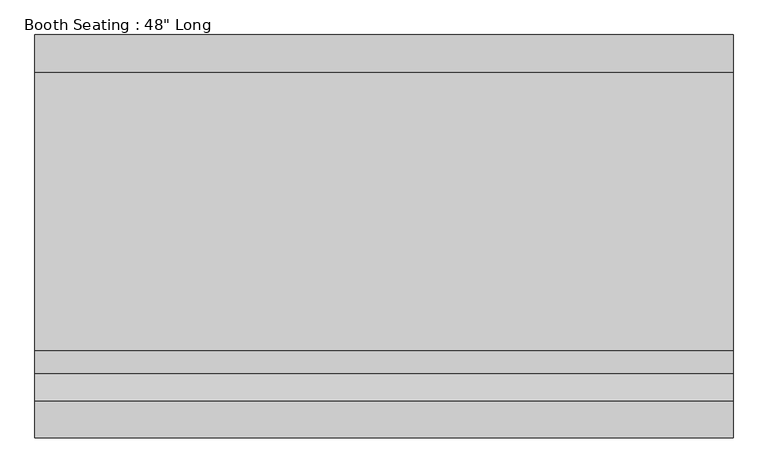
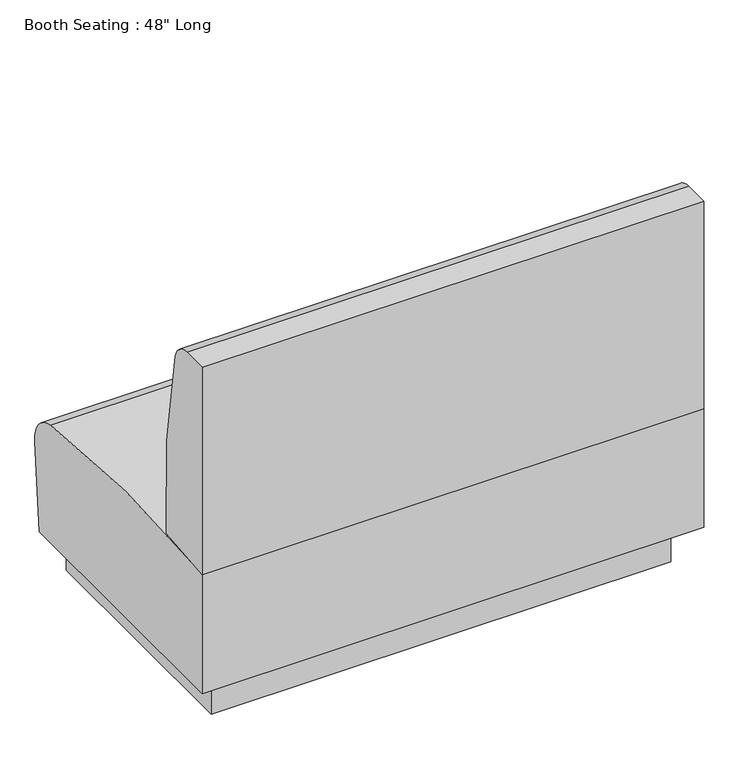
"""IFC4 building model written with IfcOpenShell, lengths in millimetres: furniture geometry."""

from ifc_helpers import new_model, si_unit, point, frame, frame_2d, origin, origin_with_axes, place, context, project, spatial, polyline, circle_curve, trimmed, segment, composite_curve, outline, extrude, source, transform, mapped, element, save


def furniture_09c69b22(model_context):
    return source(origin(), model_context, "Body", "SweptSolid", [
        extrude(outline(composite_curve([segment(polyline([(-355.6, 939.8), (-292.2747753, 939.8)]), True, "CONTINUOUS"), segment(trimmed(circle_curve(frame_2d((-292.2747753, 889.0)), 50.8), [point((-292.2747753, 939.8))], [point((-242.7504703, 900.3129667))], False, "CARTESIAN"), True, "CONTINUOUS"), segment(trimmed(circle_curve(frame_2d((-1896.6191414, 522.5154157)), 1696.4706218), [point((-242.7504703, 900.3129667))], [point((-203.2, 420.809063))], False, "CARTESIAN"), True, "CONTINUOUS"), segment(polyline([(-203.2, 420.809063), (-355.6, 406.4), (-355.6, 939.8)]), True, "CONTINUOUS")], self_intersect=False)), frame((-609.6, 0.0, 0.0), z_axis=(1.0, 0.0, 0.0), x_axis=(0.0, 1.0, 0.0)), (0.0, 0.0, 1.0), 1219.2),
        extrude(outline(composite_curve([segment(polyline([(348.6009692, 322.4116302), (330.2, 101.6), (-355.6, 101.6), (-355.6, 406.4)]), True, "CONTINUOUS"), segment(trimmed(circle_curve(frame_2d((-44.6835428, -2068.9155338)), 2494.7657275), [point((-355.6, 406.4))], [point((282.6626275, 404.2808838))], False, "CARTESIAN"), True, "CONTINUOUS"), segment(trimmed(circle_curve(frame_2d((272.6641824, 328.7396957)), 76.2), [point((282.6626275, 404.2808838))], [point((348.6009692, 322.4116302))], False, "CARTESIAN"), True, "CONTINUOUS")], self_intersect=False)), frame((-609.6, 0.0, 0.0), z_axis=(1.0, 0.0, 0.0), x_axis=(0.0, 1.0, 0.0)), (0.0, 0.0, 1.0), 1219.2),
        extrude(outline(polyline([(558.8, -304.8), (-558.8, -304.8), (-558.8, 304.8), (558.8, 304.8), (558.8, -304.8)])), origin_with_axes(), (0.0, 0.0, 1.0), 101.6),
    ])


if __name__ == "__main__":
    model = new_model("IFC4")
    model_context = context("Model", 3, world=origin())
    ifc_project = project(units=[si_unit("LENGTHUNIT", "METRE", prefix="MILLI")], contexts=[model_context])
    site = spatial("IfcSite", under=ifc_project)
    building = spatial("IfcBuilding", under=site)
    placement = place(None, origin())
    furniture_shape = furniture_09c69b22(model_context)
    element("IfcFurniture", 1, ObjectType="Booth Seating : 48\" Long", at=placement, inside=building, context=model_context, shape_type="MappedRepresentation", body=[
        mapped(furniture_shape, transform((0.0, 0.0, 0.0), x_axis=(1.0, 0.0, 0.0), y_axis=(0.0, 1.0, 0.0), z_axis=(0.0, 0.0, 1.0))),
    ])
    save(model, "model.ifc")

# Revit data of these elements
# Type "Booth Seating : 48\" Long"
#   Type Mark = "SB2"
#   Seat Height = 1' - 4"
#   Length = 4' - 0"
#   Depth = 2' - 4"
#   Back Height = 3' - 1"
#   Number of Persons = 2
#   Default Elevation = 0
# Element 1 (IfcFurniture, "Booth Seating : 48\" Long")
#   Materials on its faces: "Leather, Dark Brown", "Plastic, Opaque Black"
# Materials
#   "Leather, Dark Brown": class "Textile", colour RGB 57 45 39, transparency 0, Description = "Leather, dark brown", Cost = 0
#   "Plastic, Opaque Black": class "Plastic", colour RGB 5 5 5, transparency 0, Description = "Plastic, generic, opaque black", Cost = 0
